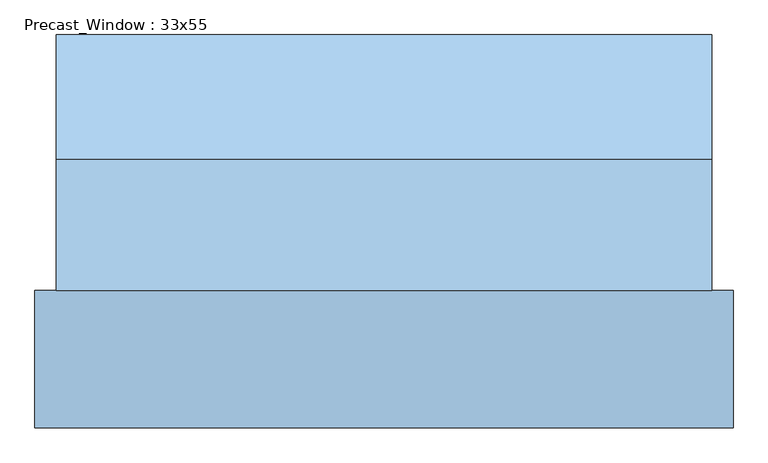
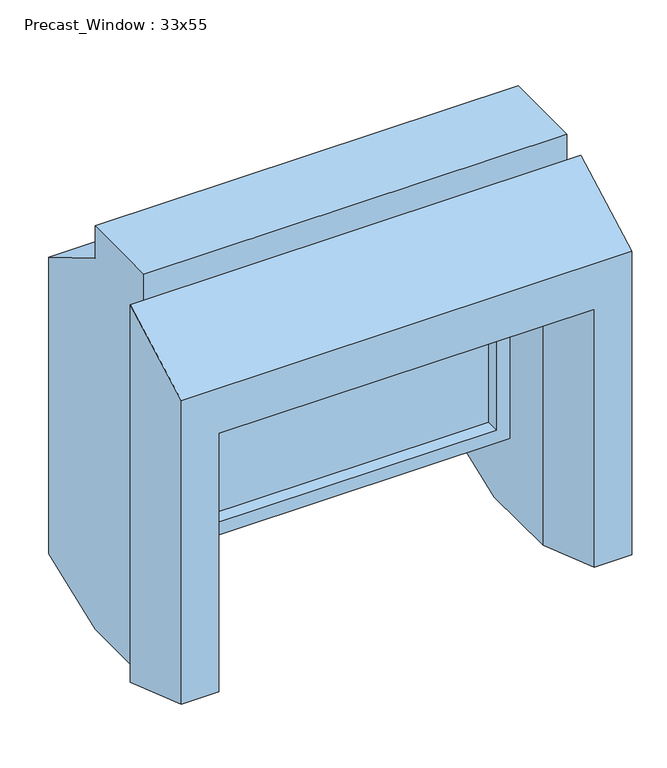
"""IFC4 building model written with IfcOpenShell, lengths in millimetres: window geometry, Precast_Window : 33x55."""

from ifc_helpers import new_model, si_unit, frame, origin, place, context, project, spatial, polyline, outline, extrude, faceted_brep, source, transform, mapped, element, save


def precast_window_33x55_fe5020ee(model_context):
    return source(origin(), model_context, "Body", "SolidModel", [
        extrude(outline(polyline([(647.7, 106.3625), (-647.7, 106.3625), (-647.7, 125.4125), (647.7, 125.4125), (647.7, 106.3625)])), frame((0.0, 0.0, 1066.8), z_axis=(0.0, 0.0, 1.0), x_axis=(1.0, 0.0, 0.0)), (0.0, 0.0, 1.0), 736.6),
        extrude(outline(polyline([(1854.2, -698.5), (1016.0, -698.5), (1016.0, 698.5), (1854.2, 698.5), (1854.2, -698.5)]), holes=[polyline([(1803.4, -647.7), (1803.4, 647.7), (1066.8, 647.7), (1066.8, -647.7), (1803.4, -647.7)])]), frame((0.0, 55.5625, 0.0), z_axis=(0.0, 1.0, 0.0), x_axis=(0.0, 0.0, 1.0)), (0.0, 0.0, 1.0), 101.6),
        faceted_brep([(838.2, -157.1625, 723.9), (838.2, -157.1625, 2209.8), (838.2, -487.3625, 2032.0), (838.2, -487.3625, 838.2), (698.5, -157.1625, 1854.2), (-698.5, -157.1625, 1854.2), (-698.5, -157.1625, 723.9), (-838.2, -157.1625, 723.9), (-838.2, -157.1625, 2209.8), (698.5, -157.1625, 723.9), (698.5, -487.3625, 838.2), (-838.2, -487.3625, 2032.0), (-838.2, -487.3625, 838.2), (-698.5, -487.3625, 838.2), (-698.5, -487.3625, 1854.2), (698.5, -487.3625, 1854.2)], [[[0, 1, 2, 3]], [[4, 5, 6, 7, 8, 1, 0, 9]], [[3, 10, 9, 0]], [[10, 3, 2, 11, 12, 13, 14, 15]], [[15, 4, 9, 10]], [[13, 12, 7, 6]], [[5, 14, 13, 6]], [[15, 14, 5, 4]], [[7, 12, 11, 8]], [[1, 8, 11, 2]]]),
        faceted_brep([(787.4, 457.2, 838.2), (787.4, 457.2, 2006.6), (787.4, 157.1625, 2184.4), (787.4, 157.1625, 2311.4), (787.4, -157.1625, 2311.4), (787.4, -157.1625, 723.9), (787.4, 157.1625, 723.9), (698.5, -157.1625, 723.9), (-787.4, -157.1625, 2311.4), (-787.4, -157.1625, 723.9), (-698.5, -157.1625, 723.9), (-698.5, -157.1625, 1854.2), (698.5, -157.1625, 1854.2), (698.5, 457.2, 1854.2), (-698.5, 457.2, 1854.2), (-698.5, 457.2, 838.2), (-787.4, 457.2, 838.2), (-787.4, 457.2, 2006.6), (698.5, 457.2, 838.2), (698.5, 157.1625, 723.9), (-787.4, 157.1625, 723.9), (-787.4, 157.1625, 2311.4), (-787.4, 157.1625, 2184.4), (-698.5, 157.1625, 723.9)], [[[0, 1, 2, 3, 4, 5, 6]], [[7, 5, 4, 8, 9, 10, 11, 12]], [[13, 14, 15, 16, 17, 1, 0, 18]], [[12, 13, 18, 19, 7]], [[16, 20, 9, 8, 21, 22, 17]], [[14, 11, 10, 23, 15]], [[12, 11, 14, 13]], [[3, 21, 8, 4]], [[2, 22, 21, 3]], [[1, 17, 22, 2]], [[6, 19, 18, 0]], [[5, 7, 19, 6]], [[10, 9, 20, 23]], [[23, 20, 16, 15]]]),
    ])


if __name__ == "__main__":
    model = new_model("IFC4")
    model_context = context("Model", 3, world=origin())
    ifc_project = project(units=[si_unit("LENGTHUNIT", "METRE", prefix="MILLI")], contexts=[model_context])
    site = spatial("IfcSite", under=ifc_project)
    building = spatial("IfcBuilding", under=site)
    placement = place(None, origin())
    precast_window_33x55_shape = precast_window_33x55_fe5020ee(model_context)
    element("IfcWindow", 1, ObjectType="Precast_Window : 33x55", at=placement, inside=building, context=model_context, shape_type="MappedRepresentation", body=[
        mapped(precast_window_33x55_shape, transform((0.0, 0.0, 0.0), x_axis=(1.0, 0.0, 0.0), y_axis=(0.0, 1.0, 0.0), z_axis=(0.0, 0.0, 1.0))),
    ])
    save(model, "model.ifc")

# Revit data of these elements
# Type "Precast_Window : 33x55"
#   Type Mark = "25"
#   Analytic Construction = "<None>"
#   Height = 2' - 9"
#   Frame Width = 0' - 2"
#   Default Sill Height = 4' - 0"
#   Width = 4' - 7"
#   Precast Material = Stucco - Plaster Cement - Taupe
#   Frame Material = Metal Trim
#   Wall Closure = (empty or 0)
# Element 1 (IfcWindow, "Precast_Window : 33x55")
#   Materials on its faces: "Stucco - Plaster Cement - Taupe", "Metal Trim", "Glass"
# Materials
#   "Stucco - Plaster Cement - Taupe": class "Generic", colour RGB 137 123 107, transparency 0, Description = "Gypsum Wall Board", Cost = 0
#   "Metal Trim": class "Wood", colour RGB 151 137 121, transparency 0, Cost = 0
#   "Glass": class "Glass", colour RGB 218 227 224, transparency 0.85, Description = "Soda Lime Glass", Cost = 0
